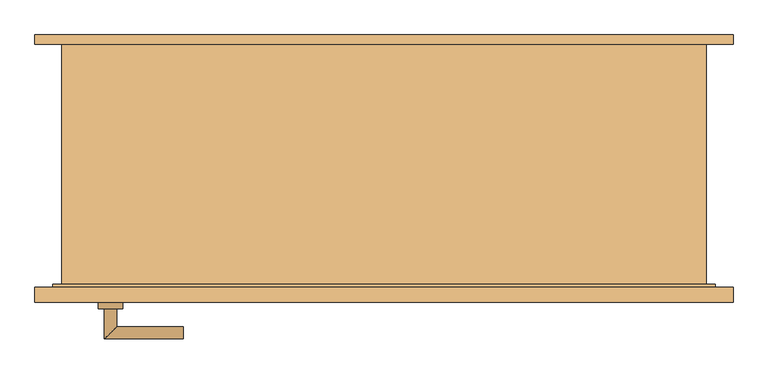
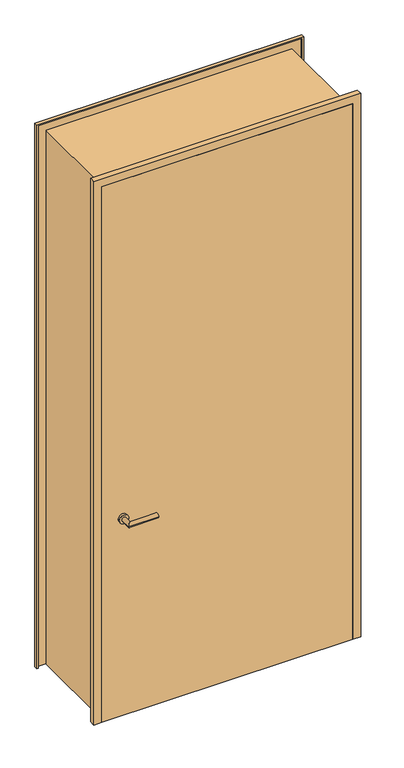
"""IFC4 building model written with IfcOpenShell, lengths in millimetres: door geometry, Drehflügel 1-flg - Stahlzarge : Glasmetalltüre 1,1 x 2,45."""

from ifc_helpers import new_model, si_unit, point, frame, frame_2d, origin, place, context, project, spatial, polyline, circle_curve, ellipse_curve, trimmed, segment, composite_curve, outline, extrude, faceted_brep, source, transform, mapped, element, save
from ifc_brep_helpers import plane_surface, cylinder_surface, advanced_brep


def door_f543baa7(model_context):
    return source(origin(), model_context, "Body", "SolidModel", [
        advanced_brep(
        [(-460.0, -189.4346141, 1000.0), (-440.0, -189.4346141, 1000.0), (-440.0, -139.4346141, 1000.0), (-460.0, -119.4346141, 1000.0), (-330.0, -119.4346141, 1000.0), (-330.0, -139.4346141, 1000.0)],
        [
            (0, 1, circle_curve(frame((-450.0, -189.4346141, 1000.0), z_axis=(0.0, -1.0, 0.0), x_axis=(1.0, 0.0, 0.0)), 10.0)),
            (1, 0, circle_curve(frame((-450.0, -189.4346141, 1000.0), z_axis=(0.0, -1.0, 0.0), x_axis=(1.0, 0.0, 0.0)), 10.0)),
            (1, 2),
            (2, 3, ellipse_curve(frame((-450.0, -129.4346141, 1000.0), z_axis=(-0.7071067811865385, -0.7071067811865565, 0.0), x_axis=(0.7071067811865563, -0.7071067811865386, 0.0)), 14.1421356, 10.0)),
            (3, 0),
            (3, 2, ellipse_curve(frame((-450.0, -129.4346141, 1000.0), z_axis=(-0.7071067811865385, -0.7071067811865565, 0.0), x_axis=(0.7071067811865563, -0.7071067811865386, 0.0)), 14.1421356, 10.0)),
            (4, 5, circle_curve(frame((-330.0, -129.4346141, 1000.0), z_axis=(1.0, 0.0, 0.0), x_axis=(0.0, -1.0, 0.0)), 10.0)),
            (5, 4, circle_curve(frame((-330.0, -129.4346141, 1000.0), z_axis=(1.0, 0.0, 0.0), x_axis=(0.0, -1.0, 0.0)), 10.0)),
            (2, 5),
            (4, 3),
        ],
        [
            plane_surface(frame((-450.0, -189.4346141, -287.7526403), z_axis=(0.0, -1.0, 0.0), x_axis=(0.0, 0.0, 1.0))),
            cylinder_surface(frame((-450.0, -189.4346141, 1000.0), z_axis=(0.0, -1.0, 0.0), x_axis=(1.0, 0.0, 0.0)), 10.0),
            plane_surface(frame((-330.0, -129.4346141, -287.7526403), z_axis=(1.0, 0.0, 0.0), x_axis=(0.0, 0.0, 1.0))),
            cylinder_surface(frame((-450.0, -129.4346141, 1000.0), z_axis=(-1.0, 0.0, 0.0), x_axis=(0.0, -1.0, 0.0)), 10.0),
        ],
        [
            (0, [[1, 2]]),
            (1, [[3, 4, 5, -2]]),
            (1, [[-5, 6, -3, -1]]),
            (2, [[7, 8]]),
            (3, [[9, -7, 10, -4]]),
            (3, [[-10, -8, -9, -6]]),
        ],
    ),
        advanced_brep(
        [(-440.0, -249.4346141, 1000.0), (-460.0, -249.4346141, 1000.0), (-460.0, -299.4346141, 1000.0), (-440.0, -279.4346141, 1000.0), (-330.0, -279.4346141, 1000.0), (-330.0, -299.4346141, 1000.0)],
        [
            (0, 1, circle_curve(frame((-450.0, -249.4346141, 1000.0), z_axis=(0.0, 1.0, 0.0), x_axis=(-1.0, 0.0, 0.0)), 10.0)),
            (1, 0, circle_curve(frame((-450.0, -249.4346141, 1000.0), z_axis=(0.0, 1.0, 0.0), x_axis=(-1.0, 0.0, 0.0)), 10.0)),
            (1, 2),
            (2, 3, ellipse_curve(frame((-450.0, -289.4346141, 1000.0), z_axis=(-0.7071067811865475, 0.7071067811865475, 0.0), x_axis=(0.7071067811865474, 0.7071067811865476, 0.0)), 14.1421356, 10.0)),
            (3, 0),
            (3, 2, ellipse_curve(frame((-450.0, -289.4346141, 1000.0), z_axis=(-0.7071067811865475, 0.7071067811865475, 0.0), x_axis=(0.7071067811865474, 0.7071067811865476, 0.0)), 14.1421356, 10.0)),
            (4, 5, circle_curve(frame((-330.0, -289.4346141, 1000.0), z_axis=(1.0, 0.0, 0.0), x_axis=(0.0, -1.0, 0.0)), 10.0)),
            (5, 4, circle_curve(frame((-330.0, -289.4346141, 1000.0), z_axis=(1.0, 0.0, 0.0), x_axis=(0.0, -1.0, 0.0)), 10.0)),
            (2, 5),
            (4, 3),
        ],
        [
            plane_surface(frame((-450.0, -249.4346141, -287.7526403), z_axis=(0.0, 1.0, 0.0), x_axis=(0.0, 0.0, 1.0))),
            cylinder_surface(frame((-450.0, -249.4346141, 1000.0), z_axis=(0.0, 1.0, 0.0), x_axis=(-1.0, 0.0, 0.0)), 10.0),
            plane_surface(frame((-330.0, -289.4346141, -287.7526403), z_axis=(1.0, 0.0, 0.0), x_axis=(0.0, 0.0, 1.0))),
            cylinder_surface(frame((-450.0, -289.4346141, 1000.0), z_axis=(-1.0, 0.0, 0.0), x_axis=(0.0, -1.0, 0.0)), 10.0),
        ],
        [
            (0, [[1, 2]]),
            (1, [[3, 4, 5, -2]]),
            (1, [[-5, 6, -3, -1]]),
            (2, [[7, 8]]),
            (3, [[9, -7, 10, -4]]),
            (3, [[-10, -8, -9, -6]]),
        ],
    ),
        extrude(outline(composite_curve([segment(trimmed(circle_curve(frame_2d((1000.0, -450.0)), 20.0), [point((1000.0, -470.0))], [point((1000.0, -430.0))], False, "CARTESIAN"), True, "CONTINUOUS"), segment(trimmed(circle_curve(frame_2d((1000.0, -450.0)), 20.0), [point((1000.0, -430.0))], [point((1000.0, -470.0))], False, "CARTESIAN"), True, "CONTINUOUS")], self_intersect=False)), frame((0.0, -189.4346141, 0.0), z_axis=(0.0, 1.0, 0.0), x_axis=(0.0, 0.0, 1.0)), (0.0, 0.0, 1.0), 10.0),
        extrude(outline(composite_curve([segment(trimmed(circle_curve(frame_2d((1000.0, -450.0)), 20.0), [point((1000.0, -470.0))], [point((1000.0, -430.0))], False, "CARTESIAN"), True, "CONTINUOUS"), segment(trimmed(circle_curve(frame_2d((1000.0, -450.0)), 20.0), [point((1000.0, -430.0))], [point((1000.0, -470.0))], False, "CARTESIAN"), True, "CONTINUOUS")], self_intersect=False)), frame((0.0, -249.4346141, 0.0), z_axis=(0.0, 1.0, 0.0), x_axis=(0.0, 0.0, 1.0)), (0.0, 0.0, 1.0), 10.0),
        extrude(outline(polyline([(540.0, -214.4346141), (540.0, -239.4346141), (-540.0, -239.4346141), (-540.0, -214.4346141), (540.0, -214.4346141)])), frame((0.0, 0.0, 100.0), z_axis=(0.0, 0.0, 1.0), x_axis=(1.0, 0.0, 0.0)), (0.0, 0.0, 1.0), 2440.0),
        faceted_brep([(574.4603207, 200.5653859, 100.0), (574.4603207, 185.5653859, 100.0), (569.4603207, 185.5653859, 100.0), (569.4603207, 195.5653859, 100.0), (530.0, 195.5653859, 100.0), (530.0, -209.4346141, 100.0), (545.0, -209.4346141, 100.0), (545.0, -234.4346141, 100.0), (569.4603207, -234.4346141, 100.0), (569.4603207, -214.4346141, 100.0), (574.4603207, -214.4346141, 100.0), (574.4603207, -239.4346141, 100.0), (540.0, -239.4346141, 100.0), (540.0, -214.4346141, 100.0), (525.0, -214.4346141, 100.0), (525.0, 200.5653859, 100.0), (525.0, 200.5653859, 2525.0), (-525.0, 200.5653859, 2525.0), (-525.0, 200.5653859, 100.0), (-574.4603207, 200.5653859, 100.0), (-574.4603207, 200.5653859, 2574.4603207), (574.4603207, 200.5653859, 2574.4603207), (525.0, -214.4346141, 2525.0), (540.0, -214.4346141, 2540.0), (-540.0, -214.4346141, 2540.0), (-540.0, -214.4346141, 100.0), (-525.0, -214.4346141, 100.0), (-525.0, -214.4346141, 2525.0), (540.0, -239.4346141, 2540.0), (574.4603207, -239.4346141, 2574.4603207), (-574.4603207, -239.4346141, 2574.4603207), (-574.4603207, -239.4346141, 100.0), (-540.0, -239.4346141, 100.0), (-540.0, -239.4346141, 2540.0), (574.4603207, -214.4346141, 2574.4603207), (569.4603207, -214.4346141, 2569.4603207), (-569.4603207, -214.4346141, 2569.4603207), (-569.4603207, -214.4346141, 100.0), (-574.4603207, -214.4346141, 100.0), (-574.4603207, -214.4346141, 2574.4603207), (569.4603207, -234.4346141, 2569.4603207), (545.0, -234.4346141, 2545.0), (-545.0, -234.4346141, 2545.0), (-545.0, -234.4346141, 100.0), (-569.4603207, -234.4346141, 100.0), (-569.4603207, -234.4346141, 2569.4603207), (545.0, -209.4346141, 2545.0), (530.0, -209.4346141, 2530.0), (-530.0, -209.4346141, 2530.0), (-530.0, -209.4346141, 100.0), (-545.0, -209.4346141, 100.0), (-545.0, -209.4346141, 2545.0), (530.0, 195.5653859, 2530.0), (569.4603207, 195.5653859, 2569.4603207), (-569.4603207, 195.5653859, 2569.4603207), (-569.4603207, 195.5653859, 100.0), (-530.0, 195.5653859, 100.0), (-530.0, 195.5653859, 2530.0), (569.4603207, 185.5653859, 2569.4603207), (574.4603207, 185.5653859, 2574.4603207), (-574.4603207, 185.5653859, 2574.4603207), (-574.4603207, 185.5653859, 100.0), (-569.4603207, 185.5653859, 100.0), (-569.4603207, 185.5653859, 2569.4603207)], [[[0, 1, 2, 3, 4, 5, 6, 7, 8, 9, 10, 11, 12, 13, 14, 15]], [[15, 16, 17, 18, 19, 20, 21, 0]], [[14, 22, 16, 15]], [[13, 23, 24, 25, 26, 27, 22, 14]], [[12, 28, 23, 13]], [[11, 29, 30, 31, 32, 33, 28, 12]], [[10, 34, 29, 11]], [[9, 35, 36, 37, 38, 39, 34, 10]], [[8, 40, 35, 9]], [[7, 41, 42, 43, 44, 45, 40, 8]], [[6, 46, 41, 7]], [[5, 47, 48, 49, 50, 51, 46, 6]], [[4, 52, 47, 5]], [[3, 53, 54, 55, 56, 57, 52, 4]], [[2, 58, 53, 3]], [[1, 59, 60, 61, 62, 63, 58, 2]], [[0, 21, 59, 1]], [[20, 19, 61, 60]], [[19, 18, 26, 25, 32, 31, 38, 37, 44, 43, 50, 49, 56, 55, 62, 61]], [[27, 26, 18, 17]], [[33, 32, 25, 24]], [[39, 38, 31, 30]], [[45, 44, 37, 36]], [[51, 50, 43, 42]], [[57, 56, 49, 48]], [[63, 62, 55, 54]], [[22, 27, 17, 16]], [[28, 33, 24, 23]], [[34, 39, 30, 29]], [[40, 45, 36, 35]], [[46, 51, 42, 41]], [[52, 57, 48, 47]], [[58, 63, 54, 53]], [[21, 20, 60, 59]]]),
    ])


if __name__ == "__main__":
    model = new_model("IFC4")
    model_context = context("Model", 3, world=origin())
    ifc_project = project(units=[si_unit("LENGTHUNIT", "METRE", prefix="MILLI")], contexts=[model_context])
    site = spatial("IfcSite", under=ifc_project)
    building = spatial("IfcBuilding", under=site)
    placement = place(None, origin())
    door_shape = door_f543baa7(model_context)
    element("IfcDoor", 1, ObjectType="Drehflügel 1-flg - Stahlzarge : Glasmetalltüre 1,1 x 2,45", at=placement, inside=building, context=model_context, shape_type="MappedRepresentation", body=[
        mapped(door_shape, transform((0.0, 0.0, 0.0), x_axis=(1.0, 0.0, 0.0), y_axis=(0.0, 1.0, 0.0), z_axis=(0.0, 0.0, 1.0))),
    ])
    save(model, "model.ifc")

# Revit data of these elements
# Type "Drehflügel 1-flg - Stahlzarge : Glasmetalltüre 1,1 x 2,45"
#   Type Mark = "25"
#   Operation = "SingleSwingRight"
#   Keynote = "16.03"
#   Analytic Construction = "Metall"
#   Thermal Resistance (R) = 0.270117 (m²·K)/W
#   Heat Transfer Coefficient (U) = 3.7021 W/(m²·K)
#   Rough Width = 1.100 m
#   Rough Height [instance default] = 2.550 m
#   Höhe Türgriff [instance default] = 0.900 m
#   Height = 2.450 m
#   Fußbodenaufbau [instance default] = 0.100 m
#   Width = 1.100 m
#   Sichtbarkeit Sturzlinien [instance default] = yes
#   Türgriff auswählen [instance default] = element 221079
#   Türgriff [instance default] = none
#   Türflügel [instance default] = none
#   Rahmen/Pfosten [instance default] = Metall - Lackiert - Grau
#   Visual Light Transmittance = 0
#   Solar Heat Gain Coefficient = 0
#   Function = (empty or 0)
#   Wall Closure = (empty or 0)
# Element 1 (IfcDoor, "Drehflügel 1-flg - Stahlzarge : Glasmetalltüre 1,1 x 2,45")
#   Türflügel = Holz - Bretterlage
#   Materials on its faces: "Metall - Lackiert - Grau", "Metall - Chrom", "Holz - Bretterlage"
# Materials
#   "Metall - Lackiert - Grau": class "Farbe 1", colour RGB 98 98 98, transparency 0, Cost = 0
#   "Metall - Chrom": class "Metall", colour RGB 247 247 247, transparency 0, Cost = 0
#   "Holz - Bretterlage": class "Holz", colour RGB 216 216 216, transparency 0, Cost = 0
